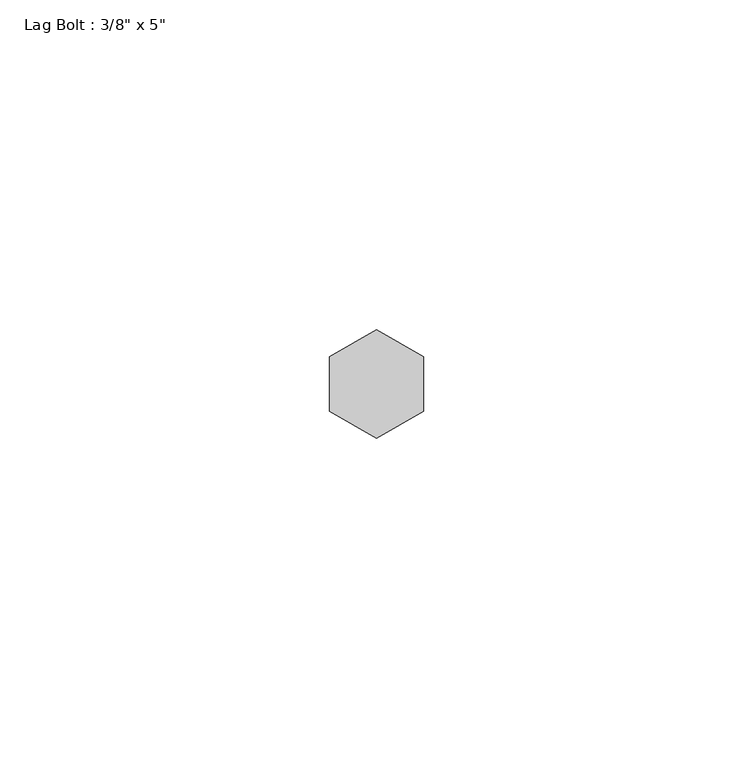
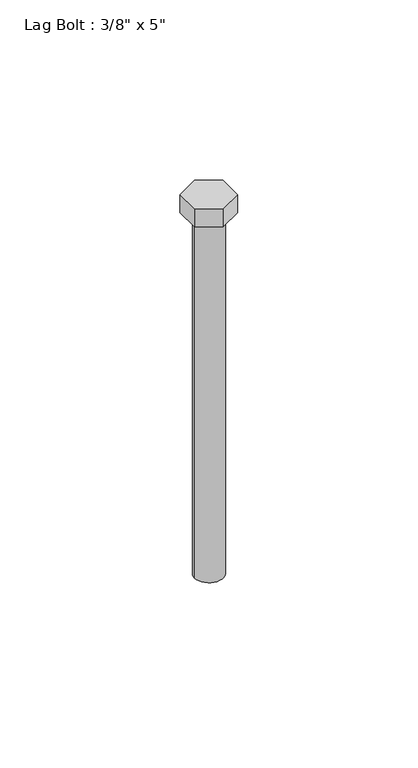
"""IFC4 building model written with IfcOpenShell, lengths in millimetres: proxy geometry."""

from ifc_helpers import new_model, si_unit, point, frame, origin, origin_with_axes, origin_2d, place, context, project, spatial, polyline, circle_curve, trimmed, segment, composite_curve, outline, extrude, source, transform, mapped, element, save


def proxy_fbd1a5cc(model_context):
    return source(origin(), model_context, "Body", "SweptSolid", [
        extrude(outline(polyline([(-7.14375, 4.124446), (0.0, 8.248892), (7.14375, 4.124446), (7.14375, -4.124446), (0.0, -8.248892), (-7.14375, -4.124446), (-7.14375, 4.124446)])), origin_with_axes(), (0.0, 0.0, 1.0), 6.35),
        extrude(outline(composite_curve([segment(trimmed(circle_curve(origin_2d(), 4.7625), [point((-4.7625, 0.0))], [point((4.7625, 0.0))], False, "CARTESIAN"), True, "CONTINUOUS"), segment(trimmed(circle_curve(origin_2d(), 4.7625), [point((4.7625, 0.0))], [point((-4.7625, 0.0))], False, "CARTESIAN"), True, "CONTINUOUS")], self_intersect=False)), frame((0.0, 0.0, -127.0), z_axis=(0.0, 0.0, 1.0), x_axis=(1.0, 0.0, 0.0)), (0.0, 0.0, 1.0), 127.0),
    ])


if __name__ == "__main__":
    model = new_model("IFC4")
    model_context = context("Model", 3, world=origin())
    ifc_project = project(units=[si_unit("LENGTHUNIT", "METRE", prefix="MILLI")], contexts=[model_context])
    site = spatial("IfcSite", under=ifc_project)
    building = spatial("IfcBuilding", under=site)
    placement = place(None, origin())
    proxy_shape = proxy_fbd1a5cc(model_context)
    element("IfcBuildingElementProxy", 1, Name="Lag Bolt : 3/8\" x 5\"", ObjectType="Lag Bolt : 3/8\" x 5\"", at=placement, inside=building, context=model_context, shape_type="MappedRepresentation", body=[
        mapped(proxy_shape, transform((0.0, 0.0, 0.0), x_axis=(1.0, 0.0, 0.0), y_axis=(0.0, 1.0, 0.0), z_axis=(0.0, 0.0, 1.0))),
    ])
    save(model, "model.ifc")

# Revit data of these elements
# Type "Lag Bolt : 3/8\" x 5\""
#   Thickness_of_Substrate [instance default] = 0' - 1"
#   Side = 0' - 0.3252"
#   Radius = 0' - 0 3/16"
#   Length = 0' - 5"
#   Head Size = 0' - 0 9/16"
#   Head Radius = 0' - 0 9/32"
#   Head Height = 0' - 0 1/4"
#   Diameter = 0' - 0 3/8"
#   Default Elevation = 4' - 0"
#   Nut_Visibility [instance default] = no
#   Bolt Material (Size) [instance default] = none
# Element 1 (IfcBuildingElementProxy, "Lag Bolt : 3/8\" x 5\"")
#   Thickness_of_Substrate = 0' - 9 1/4"
#   Bolt Material (Size) = _LAG BOTS - (SEE STRUCT. DWGS)
#   Materials on its faces: "_LAG BOTS - (SEE STRUCT. DWGS)"
# Materials
#   "_LAG BOTS - (SEE STRUCT. DWGS)": class "Metal", colour RGB 199 199 199, transparency 0, Description = "Structural steel 50ksi", Cost = 0
